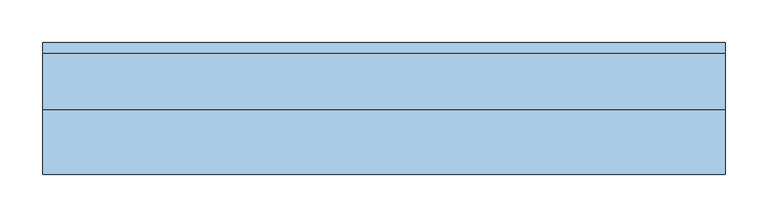
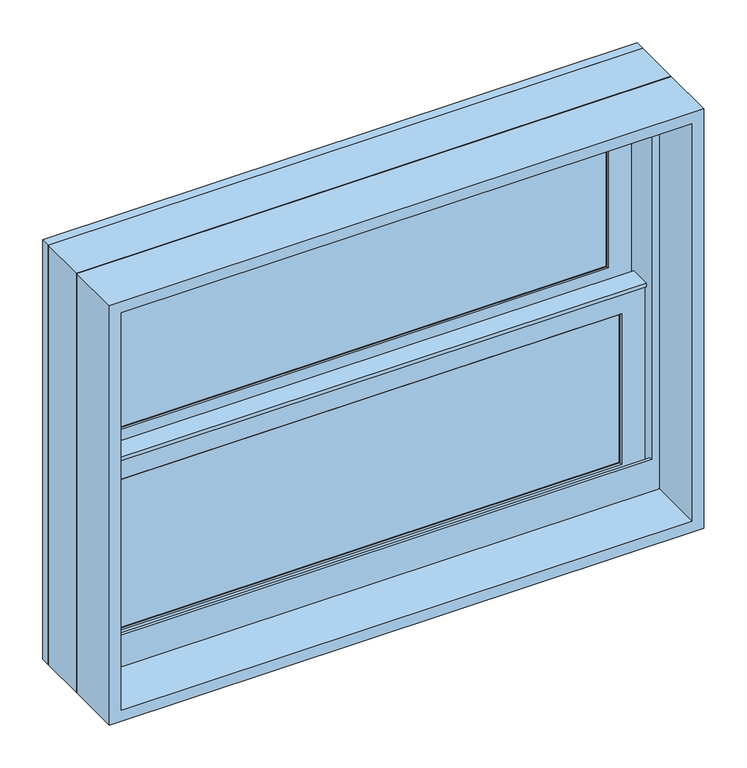
"""IFC4 building model written with IfcOpenShell, lengths in millimetres: window geometry, Window-Double_Hung-Marvin-Essential : ESDH2820."""

import ifcopenshell
import ifcopenshell.guid

model = None  # the IFC model being written
_history = None  # IfcOwnerHistory: only IFC2X3 demands one
_inside = {}  # id of a spatial element -> (the spatial element, [elements in it])
_under = {}  # id of a project, library or spatial element -> (it, [spatial elements below it])
_declared = {}  # id of a project -> (the project, [libraries it declares])
_typed = {}  # id of a type object -> (the type object, [elements of that type])
_made_of = {}  # id of a material, layer set ... -> (it, [elements and type objects made of it])


def new_model(schema):
    """Start an empty IFC model of exactly this schema.

    Asked for "IFC4X3", IfcOpenShell would pick the latest addendum, in which some entities
    have other attributes; the version numbers below select the first issue.
    IFC2X3 requires an IfcOwnerHistory on every rooted entity: one is made here for all.
    """
    global model, _history
    if schema == "IFC4X3":
        model = ifcopenshell.file(schema_version=(4, 3, 0, 0))
    else:
        model = ifcopenshell.file(schema=schema)
    _inside.clear()
    _under.clear()
    _declared.clear()
    _typed.clear()
    _made_of.clear()
    _history = None
    if model.schema == "IFC2X3":
        org = make("IfcOrganization", Name="unknown")
        user = make(
            "IfcPersonAndOrganization",
            ThePerson=make("IfcPerson", FamilyName="unknown"),
            TheOrganization=org,
        )
        app = make(
            "IfcApplication",
            ApplicationDeveloper=org,
            Version="unknown",
            ApplicationFullName="unknown",
            ApplicationIdentifier="unknown",
        )
        _history = make(
            "IfcOwnerHistory",
            OwningUser=user,
            OwningApplication=app,
            ChangeAction="ADDED",
            CreationDate=0,
        )
    return model


def make(cls, **values):
    """One entity of the class cls with the attributes given. An attribute that is None is left unset."""
    return model.create_entity(
        cls, **{name: value for name, value in values.items() if value is not None}
    )


def rooted(cls, **values):
    """An entity with a GlobalId (a new one), such as an element, a storey or a relation."""
    return make(cls, GlobalId=ifcopenshell.guid.new(), OwnerHistory=_history, **values)


def si_unit(unit_type, name, prefix=None):
    """IfcSIUnit, for example si_unit("LENGTHUNIT", "METRE", prefix="MILLI")."""
    return make("IfcSIUnit", UnitType=unit_type, Prefix=prefix, Name=name)


def assignment(units):
    """IfcUnitAssignment: the units of a project."""
    return None if units is None else make("IfcUnitAssignment", Units=units)


def point(xyz):
    """IfcCartesianPoint."""
    return None if xyz is None else make("IfcCartesianPoint", Coordinates=xyz)


def direction(xyz):
    """IfcDirection."""
    return None if xyz is None else make("IfcDirection", DirectionRatios=xyz)


def frame(location, z_axis=None, x_axis=None):
    """IfcAxis2Placement3D, a coordinate frame: its origin and axes. An axis left out is left unset."""
    return make(
        "IfcAxis2Placement3D",
        Location=point(location),
        Axis=direction(z_axis),
        RefDirection=direction(x_axis),
    )


def origin():
    """The frame at (0, 0, 0) with its axes left unset."""
    return frame((0.0, 0.0, 0.0))


def place(relative_to, where):
    """IfcLocalPlacement: puts the frame where relative to a parent placement (None: the world)."""
    return make(
        "IfcLocalPlacement", PlacementRelTo=relative_to, RelativePlacement=where
    )


def context(
    kind, dimensions, precision=None, world=None, true_north=None, identifier=None
):
    """IfcGeometricRepresentationContext, for example the 3D "Model" context."""
    return make(
        "IfcGeometricRepresentationContext",
        ContextIdentifier=identifier,
        ContextType=kind,
        CoordinateSpaceDimension=dimensions,
        Precision=precision,
        WorldCoordinateSystem=world,
        TrueNorth=true_north,
    )


def project(units=None, contexts=None):
    """IfcProject with its units and contexts."""
    return rooted(
        "IfcProject",
        Name="project",
        RepresentationContexts=contexts,
        UnitsInContext=assignment(units),
    )


def spatial(cls, under=None, at=None, **own):
    """A site, building, storey or space (cls), placed at a placement, below another one or the project."""
    s = rooted(cls, ObjectPlacement=at, **own)
    if under is not None:
        _under.setdefault(under.id(), (under, []))[1].append(s)
    return s


def polyline(points):
    """IfcPolyline through the points."""
    return make("IfcPolyline", Points=[point(p) for p in points])


def outline(outer, holes=None, kind="AREA"):
    """IfcArbitraryClosedProfileDef: a profile drawn as a closed curve; with holes, ...WithVoids."""
    if holes is None:
        return make("IfcArbitraryClosedProfileDef", ProfileType=kind, OuterCurve=outer)
    return make(
        "IfcArbitraryProfileDefWithVoids",
        ProfileType=kind,
        OuterCurve=outer,
        InnerCurves=holes,
    )


def extrude(swept, where, along, depth):
    """IfcExtrudedAreaSolid: the profile swept, set in the frame where, extruded along a direction by depth."""
    return make(
        "IfcExtrudedAreaSolid",
        SweptArea=swept,
        Position=where,
        ExtrudedDirection=direction(along),
        Depth=depth,
    )


def faces_of(points, faces, orient=None, outer=None):
    """IfcFace entities. A face is a list of loops; a loop is a list of indices into points, from 0.

    orient and outer hold one flag for each loop. By default every Orientation is true, the
    first loop of a face is its IfcFaceOuterBound and the others are IfcFaceBound.
    """
    made = []
    for i, loops in enumerate(faces):
        bounds = []
        for j, loop in enumerate(loops):
            is_outer = j == 0 if outer is None else outer[i][j]
            bounds.append(
                make(
                    "IfcFaceOuterBound" if is_outer else "IfcFaceBound",
                    Bound=make("IfcPolyLoop", Polygon=[points[k] for k in loop]),
                    Orientation=True if orient is None else orient[i][j],
                )
            )
        made.append(make("IfcFace", Bounds=bounds))
    return made


def faceted_brep(points, faces, orient=None, outer=None, voids=None):
    """IfcFacetedBrep: a solid bounded by flat faces; with voids (closed shells), ...WithVoids."""
    shared = [point(p) for p in points]
    hull = make("IfcClosedShell", CfsFaces=faces_of(shared, faces, orient, outer))
    if voids is None:
        return make("IfcFacetedBrep", Outer=hull)
    return make(
        "IfcFacetedBrepWithVoids",
        Outer=hull,
        Voids=[
            make(cls, CfsFaces=faces_of(shared, fs, o, b)) for cls, fs, o, b in voids
        ],
    )


def shape(context_of_items, identifier, shape_type, items):
    """IfcShapeRepresentation: the items that make up one representation, for example the "Body"."""
    return make(
        "IfcShapeRepresentation",
        ContextOfItems=context_of_items,
        RepresentationIdentifier=identifier,
        RepresentationType=shape_type,
        Items=items,
    )


def source(mapping_origin, context_of_items, identifier, shape_type, items):
    """IfcRepresentationMap: a shape defined once, which mapped items show again and again."""
    return make(
        "IfcRepresentationMap",
        MappingOrigin=mapping_origin,
        MappedRepresentation=shape(context_of_items, identifier, shape_type, items),
    )


def transform(
    local_origin,
    x_axis=None,
    y_axis=None,
    z_axis=None,
    scale=None,
    scale2=None,
    scale3=None,
    uniform=True,
):
    """IfcCartesianTransformationOperator3D, or its non-uniform kind. x_axis, y_axis, z_axis: its Axis1, 2, 3."""
    if uniform:
        return make(
            "IfcCartesianTransformationOperator3D",
            Axis1=direction(x_axis),
            Axis2=direction(y_axis),
            LocalOrigin=point(local_origin),
            Scale=scale,
            Axis3=direction(z_axis),
        )
    return make(
        "IfcCartesianTransformationOperator3DnonUniform",
        Axis1=direction(x_axis),
        Axis2=direction(y_axis),
        LocalOrigin=point(local_origin),
        Scale=scale,
        Axis3=direction(z_axis),
        Scale2=scale2,
        Scale3=scale3,
    )


def mapped(mapping_source, mapping_target):
    """IfcMappedItem: shows the shape of a source again, moved by a transform."""
    return make(
        "IfcMappedItem", MappingSource=mapping_source, MappingTarget=mapping_target
    )


def made_of(thing, what):
    """Note that an element or type object is made of a material, layer set ...; save() writes the relation."""
    if what is not None:
        _made_of.setdefault(what.id(), (what, []))[1].append(thing)
    return thing


def element(
    cls,
    number,
    at=None,
    inside=None,
    cuts=None,
    type_object=None,
    material=None,
    context=None,
    identifier="Body",
    shape_type=None,
    held_by="IfcProductDefinitionShape",
    body=None,
    shapes=None,
    **own,
):
    """One element of the class cls, such as IfcWall. Its Tag is "e" and its number.

    at: its placement. inside: the storey or other place that contains it. cuts: it is an
    opening in that element (IfcRelVoidsElement). A single representation is given by context,
    identifier, shape_type and body (its items); several are given by shapes. held_by: the class
    of the entity that holds the representations. save() writes the other relations.
    """
    e = rooted(cls, Tag="e%d" % number, ObjectPlacement=at, **own)
    if body is not None:
        shapes = [shape(context, identifier, shape_type, body)]
    if shapes is not None:
        e.Representation = make(held_by, Representations=shapes)
    if inside is not None:
        _inside.setdefault(inside.id(), (inside, []))[1].append(e)
    if cuts is not None:
        rooted(
            "IfcRelVoidsElement", RelatingBuildingElement=cuts, RelatedOpeningElement=e
        )
    if type_object is not None:
        _typed.setdefault(type_object.id(), (type_object, []))[1].append(e)
    return made_of(e, material)


def aggregate(whole, parts):
    """IfcRelAggregates: a whole, such as a stair, and the parts it consists of."""
    return rooted("IfcRelAggregates", RelatingObject=whole, RelatedObjects=parts)


def save(model, path):
    """Write the relations noted so far, then the file.

    IfcRelAggregates (storeys below a building ...), IfcRelContainedInSpatialStructure (elements
    in a storey), IfcRelDefinesByType, IfcRelAssociatesMaterial and IfcRelDeclares: one each for
    every whole, place, type object, material and project.
    """
    for whole, parts in _under.values():
        aggregate(whole, parts)
    for where, things in _inside.values():
        rooted(
            "IfcRelContainedInSpatialStructure",
            RelatedElements=things,
            RelatingStructure=where,
        )
    for kind, things in _typed.values():
        rooted("IfcRelDefinesByType", RelatedObjects=things, RelatingType=kind)
    for what, things in _made_of.values():
        rooted("IfcRelAssociatesMaterial", RelatedObjects=things, RelatingMaterial=what)
    for by, libraries in _declared.values():
        rooted("IfcRelDeclares", RelatingContext=by, RelatedDefinitions=libraries)
    model.write(path)


def window_5b86a6a2(model_context):
    return source(origin(), model_context, "Body", "SolidModel", [
        extrude(outline(polyline([(123.825, 20.6375), (123.825, 15.875), (104.775, 15.875), (104.775, 20.6375), (123.825, 20.6375)])), frame((0.0, 0.0, 1898.65), z_axis=(0.0, 0.0, 1.0), x_axis=(1.0, 0.0, 0.0)), (0.0, 0.0, 1.0), 222.25),
        extrude(outline(polyline([(-104.775, 20.6375), (-104.775, 15.875), (-123.825, 15.875), (-123.825, 20.6375), (-104.775, 20.6375)])), frame((0.0, 0.0, 1898.65), z_axis=(0.0, 0.0, 1.0), x_axis=(1.0, 0.0, 0.0)), (0.0, 0.0, 1.0), 222.25),
        extrude(outline(polyline([(342.9, 20.6375), (342.9, 15.875), (-342.9, 15.875), (-342.9, 20.6375), (342.9, 20.6375)])), frame((0.0, 0.0, 2000.25), z_axis=(0.0, 0.0, 1.0), x_axis=(1.0, 0.0, 0.0)), (0.0, 0.0, 1.0), 19.05),
        extrude(outline(polyline([(-123.825, 46.83125), (-123.825, 51.59375), (-104.775, 51.59375), (-104.775, 46.83125), (-123.825, 46.83125)])), frame((0.0, 0.0, 2159.0), z_axis=(0.0, 0.0, 1.0), x_axis=(1.0, 0.0, 0.0)), (0.0, 0.0, 1.0), 222.25),
        extrude(outline(polyline([(104.775, 46.83125), (104.775, 51.59375), (123.825, 51.59375), (123.825, 46.83125), (104.775, 46.83125)])), frame((0.0, 0.0, 2159.0), z_axis=(0.0, 0.0, 1.0), x_axis=(1.0, 0.0, 0.0)), (0.0, 0.0, 1.0), 222.25),
        extrude(outline(polyline([(-342.9, 46.83125), (-342.9, 51.59375), (342.9, 51.59375), (342.9, 46.83125), (-342.9, 46.83125)])), frame((0.0, 0.0, 2260.6), z_axis=(0.0, 0.0, 1.0), x_axis=(1.0, 0.0, 0.0)), (0.0, 0.0, 1.0), 19.05),
        extrude(outline(polyline([(123.825, 20.6375), (104.775, 20.6375), (104.775, 25.4), (123.825, 25.4), (123.825, 20.6375)])), frame((0.0, 0.0, 1898.65), z_axis=(0.0, 0.0, 1.0), x_axis=(1.0, 0.0, 0.0)), (0.0, 0.0, 1.0), 222.25),
        extrude(outline(polyline([(-104.775, 20.6375), (-123.825, 20.6375), (-123.825, 25.4), (-104.775, 25.4), (-104.775, 20.6375)])), frame((0.0, 0.0, 1898.65), z_axis=(0.0, 0.0, 1.0), x_axis=(1.0, 0.0, 0.0)), (0.0, 0.0, 1.0), 222.25),
        extrude(outline(polyline([(342.9, 20.6375), (-342.9, 20.6375), (-342.9, 25.4), (342.9, 25.4), (342.9, 20.6375)])), frame((0.0, 0.0, 2000.25), z_axis=(0.0, 0.0, 1.0), x_axis=(1.0, 0.0, 0.0)), (0.0, 0.0, 1.0), 19.05),
        extrude(outline(polyline([(-123.825, 56.35625), (-104.775, 56.35625), (-104.775, 51.59375), (-123.825, 51.59375), (-123.825, 56.35625)])), frame((0.0, 0.0, 2159.0), z_axis=(0.0, 0.0, 1.0), x_axis=(1.0, 0.0, 0.0)), (0.0, 0.0, 1.0), 222.25),
        extrude(outline(polyline([(104.775, 56.35625), (123.825, 56.35625), (123.825, 51.59375), (104.775, 51.59375), (104.775, 56.35625)])), frame((0.0, 0.0, 2159.0), z_axis=(0.0, 0.0, 1.0), x_axis=(1.0, 0.0, 0.0)), (0.0, 0.0, 1.0), 222.25),
        extrude(outline(polyline([(-342.9, 56.35625), (342.9, 56.35625), (342.9, 51.59375), (-342.9, 51.59375), (-342.9, 56.35625)])), frame((0.0, 0.0, 2260.6), z_axis=(0.0, 0.0, 1.0), x_axis=(1.0, 0.0, 0.0)), (0.0, 0.0, 1.0), 19.05),
        faceted_brep([(-369.8875, 5.6780605, 2150.9351748), (-369.8875, 5.6780605, 2146.3), (369.8875, 5.6780605, 2146.3), (369.8875, 5.6780605, 2150.9351748), (-369.8875, 34.8118605, 2150.9351748), (369.8875, 34.8118605, 2150.9351748), (369.8875, 34.8118605, 2146.3), (-369.8875, 34.8118605, 2146.3), (-369.8875, 30.1625, 2146.3), (-369.8875, 30.1625, 1871.6625), (-369.8875, 8.9241104, 1871.6625), (-369.8875, 8.9241104, 2146.3), (369.8875, 8.9241104, 2146.3), (369.8875, 30.1625, 2146.3), (369.8875, 8.9241104, 1871.6625), (369.8875, 30.1625, 1871.6625), (-354.0034752, 11.90625, 2132.0034752), (-354.0034752, 30.1625, 2132.0034752), (354.0034752, 30.1625, 2132.0034752), (354.0034752, 11.90625, 2132.0034752), (-337.34375, 10.4662439, 2115.34375), (-337.34375, 11.90625, 2115.34375), (337.34375, 11.90625, 2115.34375), (337.34375, 10.4662439, 2115.34375), (338.8858834, 8.9241104, 2116.8858834), (-338.8858834, 8.9241104, 2116.8858834), (354.0034752, 30.1625, 1887.5465248), (354.0034752, 11.90625, 1887.5465248), (337.34375, 11.90625, 1904.20625), (337.34375, 10.4662439, 1904.20625), (338.8858834, 8.9241104, 1902.6641166), (-354.0034752, 30.1625, 1887.5465248), (-354.0034752, 11.90625, 1887.5465248), (-337.34375, 11.90625, 1904.20625), (-337.34375, 10.4662439, 1904.20625), (-338.8858834, 8.9241104, 1902.6641166)], [[[0, 1, 2, 3]], [[4, 5, 6, 7]], [[1, 0, 4, 7, 8, 9, 10, 11]], [[2, 1, 11, 12]], [[7, 6, 13, 8]], [[3, 2, 12, 14, 15, 13, 6, 5]], [[0, 3, 5, 4]], [[16, 17, 18, 19]], [[20, 21, 22, 23]], [[20, 23, 24, 25]], [[19, 18, 26, 27]], [[23, 22, 28, 29]], [[24, 23, 29, 30]], [[27, 26, 31, 32]], [[29, 28, 33, 34]], [[30, 29, 34, 35]], [[15, 14, 10, 9]], [[15, 9, 8, 13], [18, 17, 31, 26]], [[17, 16, 32, 31]], [[16, 19, 27, 32], [22, 21, 33, 28]], [[21, 20, 34, 33]], [[20, 25, 35, 34]], [[10, 14, 12, 11], [25, 24, 30, 35]]]),
        extrude(outline(polyline([(38.5955581, 2132.0125), (33.5778968, 2132.0125), (33.5778968, 2133.6), (39.9405976, 2133.6), (39.9405976, 2132.0125), (61.515625, 2132.0125), (47.6307501, 2128.6975159), (38.5955581, 2128.6975159), (38.5955581, 2132.0125)])), frame((-369.8875, 0.0, 0.0), z_axis=(1.0, 0.0, 0.0), x_axis=(0.0, 1.0, 0.0)), (0.0, 0.0, 1.0), 739.775),
        faceted_brep([(400.05, 0.0, 1841.5), (400.05, 0.0, 2438.4), (-400.05, 0.0, 2438.4), (-400.05, 0.0, 1841.5), (373.85625, 0.0, 1902.61875), (-373.85625, 0.0, 1902.61875), (-373.85625, 0.0, 2412.20625), (373.85625, 0.0, 2412.20625), (373.85625, 3.96875, 1841.5), (-373.85625, 3.96875, 1841.5), (-373.85625, 3.96875, 1902.61875), (373.85625, 3.96875, 1902.61875), (-400.05, 65.6828125, 1841.5), (-373.85625, 65.6828125, 1841.5), (373.85625, 65.6828125, 1841.5), (400.05, 65.6828125, 1841.5), (-400.05, 65.6828125, 2438.4), (400.05, 65.6828125, 2438.4), (373.85625, 65.6828125, 2412.20625), (-373.85625, 65.6828125, 2412.20625)], [[[0, 1, 2, 3], [4, 5, 6, 7]], [[8, 9, 10, 11]], [[5, 4, 11, 10]], [[0, 3, 12, 13, 9, 8, 14, 15]], [[13, 12, 16, 17, 15, 14, 18, 19]], [[13, 19, 6, 5, 10, 9]], [[7, 6, 19, 18]], [[18, 14, 8, 11, 4, 7]], [[1, 0, 15, 17]], [[2, 1, 17, 16]], [[3, 2, 16, 12]]]),
        faceted_brep([(373.85625, 30.1625, 2139.95), (372.26875, 30.1625, 2139.95), (372.26875, 30.1625, 1865.8544613), (373.85625, 30.1625, 1865.8544613), (-372.26875, 30.1625, 2139.95), (-373.85625, 30.1625, 2139.95), (-373.85625, 30.1625, 1865.8544613), (-372.26875, 30.1625, 1865.8544613), (372.26875, 63.5, 2139.95), (373.85625, 63.5, 2139.95), (373.85625, 63.5, 1859.3743077), (372.26875, 63.5, 1859.3743077), (-373.85625, 63.5, 2139.95), (-372.26875, 63.5, 2139.95), (-372.26875, 63.5, 1859.3743077), (-373.85625, 63.5, 1859.3743077), (385.1108932, 3.96875, 1870.9460105), (385.1108932, 3.96875, 1841.5), (385.1108932, 65.6828125, 1841.5), (385.1108932, 65.6828125, 1858.950012), (-385.1108932, 3.96875, 1841.5), (-385.1108932, 3.96875, 1870.9460105), (-385.1108932, 65.6828125, 1858.950012), (-385.1108932, 65.6828125, 1841.5), (385.1108932, 78.58125, 1856.4428097), (-385.1108932, 78.58125, 1856.4428097), (-383.0971252, 68.2348864, 1858.4539391), (-365.13135, 68.2348864, 1858.4539391), (-365.13135, 65.6828125, 1858.950012), (365.13135, 65.6828125, 1858.950012), (365.13135, 68.2348864, 1858.4539391), (383.0971252, 68.2348864, 1858.4539391), (-400.05, 65.6828125, 1841.5), (-400.05, 78.5948249, 1841.5), (400.05, 78.5948249, 1841.5), (400.05, 65.6828125, 1841.5), (-400.05, 78.58125, 2438.4), (400.05, 78.58125, 2438.4), (385.1108932, 78.58125, 2423.4608932), (-385.1108932, 78.58125, 2423.4608932), (-400.05, 65.6828125, 2438.4), (-383.0971252, 68.2348864, 2421.4471252), (383.0971252, 68.2348864, 2421.4471252), (365.13135, 68.2348864, 2403.48135), (-365.13135, 68.2348864, 2403.48135), (-365.13135, 65.6828125, 2403.48135), (365.13135, 65.6828125, 2403.48135), (400.05, 65.6828125, 2438.4)], [[[0, 1, 2, 3]], [[4, 5, 6, 7]], [[8, 9, 10, 11]], [[12, 13, 14, 15]], [[1, 8, 11, 2]], [[9, 0, 3, 10]], [[1, 0, 9, 8]], [[5, 4, 13, 12]], [[5, 12, 15, 6]], [[13, 4, 7, 14]], [[16, 17, 18, 19]], [[20, 21, 22, 23]], [[24, 25, 26, 27, 28, 22, 21, 16, 19, 29, 30, 31], [3, 2, 11, 10], [7, 6, 15, 14]], [[17, 16, 21, 20]], [[17, 20, 23, 32, 33, 34, 35, 18]], [[34, 33, 36, 37], [25, 24, 38, 39]], [[33, 32, 40, 36]], [[39, 41, 26, 25]], [[41, 42, 31, 30, 43, 44, 27, 26]], [[44, 45, 28, 27]], [[40, 32, 23, 22, 28, 45, 46, 29, 19, 18, 35, 47]], [[36, 40, 47, 37]], [[39, 38, 42, 41]], [[44, 43, 46, 45]], [[34, 37, 47, 35]], [[42, 38, 24, 31]], [[46, 43, 30, 29]]]),
        extrude(outline(polyline([(350.04375, 11.90625), (-350.04375, 11.90625), (-350.04375, 15.08125), (350.04375, 15.08125), (350.04375, 11.90625)])), frame((0.0, 0.0, 1891.50625), z_axis=(0.0, 0.0, 1.0), x_axis=(1.0, 0.0, 0.0)), (0.0, 0.0, 1.0), 236.5375),
        extrude(outline(polyline([(350.04375, 42.8625), (-350.04375, 42.8625), (-350.04375, 46.0375), (350.04375, 46.0375), (350.04375, 42.8625)])), frame((0.0, 0.0, 2151.85625), z_axis=(0.0, 0.0, 1.0), x_axis=(1.0, 0.0, 0.0)), (0.0, 0.0, 1.0), 236.5375),
        faceted_brep([(-337.34375, 31.194477, 2115.34375), (-338.8858834, 32.7366104, 2116.8858834), (338.8858834, 32.7366104, 2116.8858834), (337.34375, 31.194477, 2115.34375), (-337.34375, 30.1625, 2115.34375), (337.34375, 30.1625, 2115.34375), (-369.8875, 32.7366104, 2147.8875), (-369.8875, 30.1625, 2147.8875), (369.8875, 30.1625, 2147.8875), (369.8875, 32.7366104, 2147.8875), (338.8858834, 32.7366104, 1902.6641166), (337.34375, 31.194477, 1904.20625), (337.34375, 30.1625, 1904.20625), (369.8875, 30.1625, 1871.6625), (369.8875, 32.7366104, 1871.6625), (-338.8858834, 32.7366104, 1902.6641166), (-337.34375, 31.194477, 1904.20625), (-337.34375, 30.1625, 1904.20625), (-369.8875, 30.1625, 1871.6625), (-369.8875, 32.7366104, 1871.6625)], [[[0, 1, 2, 3]], [[4, 0, 3, 5]], [[6, 7, 8, 9]], [[3, 2, 10, 11]], [[5, 3, 11, 12]], [[9, 8, 13, 14]], [[11, 10, 15, 16]], [[12, 11, 16, 17]], [[14, 13, 18, 19]], [[9, 14, 19, 6], [1, 15, 10, 2]], [[16, 15, 1, 0]], [[17, 16, 0, 4]], [[7, 18, 13, 8], [5, 12, 17, 4]], [[19, 18, 7, 6]]]),
        faceted_brep([(-354.0034752, 42.8625, 2392.3534752), (-354.0034752, 61.11875, 2392.3534752), (354.0034752, 61.11875, 2392.3534752), (354.0034752, 42.8625, 2392.3534752), (-337.34375, 41.4224939, 2375.69375), (-337.34375, 42.8625, 2375.69375), (337.34375, 42.8625, 2375.69375), (337.34375, 41.4224939, 2375.69375), (-338.8858834, 39.8803604, 2377.2358834), (338.8858834, 39.8803604, 2377.2358834), (-369.8875, 61.11875, 2408.2375), (-369.8875, 39.8803604, 2408.2375), (369.8875, 39.8803604, 2408.2375), (369.8875, 61.11875, 2408.2375), (354.0034752, 61.11875, 2147.8965248), (354.0034752, 42.8625, 2147.8965248), (337.34375, 42.8625, 2164.55625), (337.34375, 41.4224939, 2164.55625), (338.8858834, 39.8803604, 2163.0141166), (369.8875, 39.8803604, 2132.0125), (369.8875, 61.11875, 2132.0125), (-354.0034752, 61.11875, 2147.8965248), (-354.0034752, 42.8625, 2147.8965248), (-337.34375, 42.8625, 2164.55625), (-337.34375, 41.4224939, 2164.55625), (-338.8858834, 39.8803604, 2163.0141166), (-369.8875, 39.8803604, 2132.0125), (-369.8875, 61.11875, 2132.0125)], [[[0, 1, 2, 3]], [[4, 5, 6, 7]], [[8, 4, 7, 9]], [[10, 11, 12, 13]], [[3, 2, 14, 15]], [[7, 6, 16, 17]], [[9, 7, 17, 18]], [[13, 12, 19, 20]], [[15, 14, 21, 22]], [[17, 16, 23, 24]], [[18, 17, 24, 25]], [[20, 19, 26, 27]], [[13, 20, 27, 10], [1, 21, 14, 2]], [[22, 21, 1, 0]], [[3, 15, 22, 0], [5, 23, 16, 6]], [[24, 23, 5, 4]], [[25, 24, 4, 8]], [[11, 26, 19, 12], [9, 18, 25, 8]], [[27, 26, 11, 10]]]),
        faceted_brep([(-369.8875, 61.11875, 2132.0125), (-369.8875, 63.6928604, 2132.0125), (369.8875, 63.6928604, 2132.0125), (369.8875, 61.11875, 2132.0125), (-337.34375, 62.150727, 2164.55625), (-337.34375, 61.11875, 2164.55625), (337.34375, 61.11875, 2164.55625), (337.34375, 62.150727, 2164.55625), (-338.8858834, 63.6928604, 2163.0141166), (338.8858834, 63.6928604, 2163.0141166), (369.8875, 63.6928604, 2408.2375), (369.8875, 61.11875, 2408.2375), (337.34375, 61.11875, 2375.69375), (337.34375, 62.150727, 2375.69375), (338.8858834, 63.6928604, 2377.2358834), (-369.8875, 63.6928604, 2408.2375), (-369.8875, 61.11875, 2408.2375), (-337.34375, 61.11875, 2375.69375), (-337.34375, 62.150727, 2375.69375), (-338.8858834, 63.6928604, 2377.2358834)], [[[0, 1, 2, 3]], [[4, 5, 6, 7]], [[8, 4, 7, 9]], [[3, 2, 10, 11]], [[7, 6, 12, 13]], [[9, 7, 13, 14]], [[11, 10, 15, 16]], [[13, 12, 17, 18]], [[14, 13, 18, 19]], [[16, 15, 1, 0]], [[3, 11, 16, 0], [5, 17, 12, 6]], [[18, 17, 5, 4]], [[19, 18, 4, 8]], [[1, 15, 10, 2], [9, 14, 19, 8]]]),
        extrude(outline(polyline([(350.04375, 26.19375), (-350.04375, 26.19375), (-350.04375, 30.1625), (350.04375, 30.1625), (350.04375, 26.19375)])), frame((0.0, 0.0, 1891.50625), z_axis=(0.0, 0.0, 1.0), x_axis=(1.0, 0.0, 0.0)), (0.0, 0.0, 1.0), 236.5375),
        extrude(outline(polyline([(350.04375, 57.15), (-350.04375, 57.15), (-350.04375, 61.11875), (350.04375, 61.11875), (350.04375, 57.15)])), frame((0.0, 0.0, 2151.85625), z_axis=(0.0, 0.0, 1.0), x_axis=(1.0, 0.0, 0.0)), (0.0, 0.0, 1.0), 236.5375),
        extrude(outline(polyline([(2438.4, 400.05), (2438.4, -400.05), (1841.5, -400.05), (1841.5, 400.05), (2438.4, 400.05)]), holes=[polyline([(2422.525, 384.175), (1857.375, 384.175), (1857.375, -384.175), (2422.525, -384.175), (2422.525, 384.175)])]), frame((0.0, -76.2, 0.0), z_axis=(0.0, 1.0, 0.0), x_axis=(0.0, 0.0, 1.0)), (0.0, 0.0, 1.0), 75.40625),
    ])


if __name__ == "__main__":
    model = new_model("IFC4")
    model_context = context("Model", 3, world=origin())
    ifc_project = project(units=[si_unit("LENGTHUNIT", "METRE", prefix="MILLI")], contexts=[model_context])
    site = spatial("IfcSite", under=ifc_project)
    building = spatial("IfcBuilding", under=site)
    placement = place(None, origin())
    window_shape = window_5b86a6a2(model_context)
    element("IfcWindow", 1, ObjectType="Window-Double_Hung-Marvin-Essential : ESDH2820", at=placement, inside=building, context=model_context, shape_type="MappedRepresentation", body=[
        mapped(window_shape, transform((0.0, 0.0, 0.0), x_axis=(1.0, 0.0, 0.0), y_axis=(0.0, 1.0, 0.0), z_axis=(0.0, 0.0, 1.0))),
    ])
    save(model, "model.ifc")

# Revit data of these elements
# Type "Window-Double_Hung-Marvin-Essential : ESDH2820"
#   Type Mark = "22"
#   Window Type = "Essential Double Hung"
#   Product data url = "https://bimobject.com/marvin-windows-and-doors/product/marvin-dhwau"
#   Product Guid = "c4a96547-874c-4385-91dc-a058adc19d98"
#   Frame = "All Ultrex"
#   Egress Window = "No"
#   URL = "www.marvin.com"
#   Model = "ESDH2820"
#   Manufacturer = "Marvin Windows and Doors"
#   Label Egress = ""
#   Glass Type = "IG Low E II with Argon"
#   Design Pressure = "DP50"
#   Description = "3224 DBHG"
#   Analytic Construction = "<None>"
#   Prairie Corner Width = 0' - 4"
#   Prairie Corner Height = 0' - 4"
#   Egress Width = 2' - 4 9/16"
#   Egress Height = 0' - 7 27/128"
#   Rough Width = 2' - 8"
#   Rough Height = 2' - 0"
#   Nominal Width = 2' - 8"
#   Nominal Height = 2' - 0"
#   Inset to Installation Flange [instance default] = 0' - 1"
#   Height = 1' - 11 1/2"
#   Egress Area = 1.43029 SF
#   Default Head Height = 8' - 0"
#   Width = 2' - 7 1/2"
#   Daylight Area = 3.06668 SF
#   DLO Width = 2' - 2 9/16"
#   DLO Height = 0' - 8 5/16"
#   Muntins Top Sash = yes
#   Lites Wide Top Sash = 3
#   Lites Wide Bottom Sash = 3
#   Lites High Top Sash = 2
#   Lites High Bottom Sash = 2
#   Lite Cut Prairie 9 = no
#   Lite Cut HV Grid = yes
#   Muntins Bottom Sash = yes
#   Label Visibility = no
#   Jamb Extension Visibility = yes
#   Edition number = 1
#   Interior Material = Ultrex-Marvin-Stonewhite
#   Glazing Material = Glass-Marvin-IG Low E II with Argon
#   Cladding Material = Ultrex-Marvin-Pebblegray
#   Wall Closure = (empty or 0)
#   Assembly Code = ""
# Element 1 (IfcWindow, "Window-Double_Hung-Marvin-Essential : ESDH2820")
#   Materials on its faces: "Ultrex-Marvin-Pebblegray", "Ultrex-Marvin-Stonewhite", "Glass-Marvin-IG Low E II with Argon"
# Materials
#   "Ultrex-Marvin-Stonewhite": class "Paint", colour RGB 250 251 245, transparency 0
#   "Glass-Marvin-IG Low E II with Argon": class "Glass", colour RGB 0 128 192, transparency 0.85
#   "Ultrex-Marvin-Pebblegray": class "Paint", colour RGB 189 185 173, transparency 0
